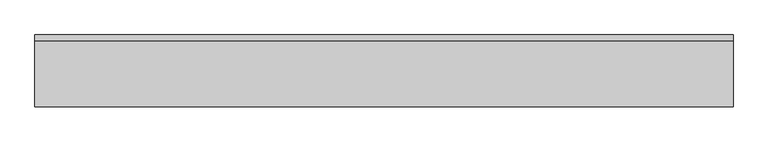
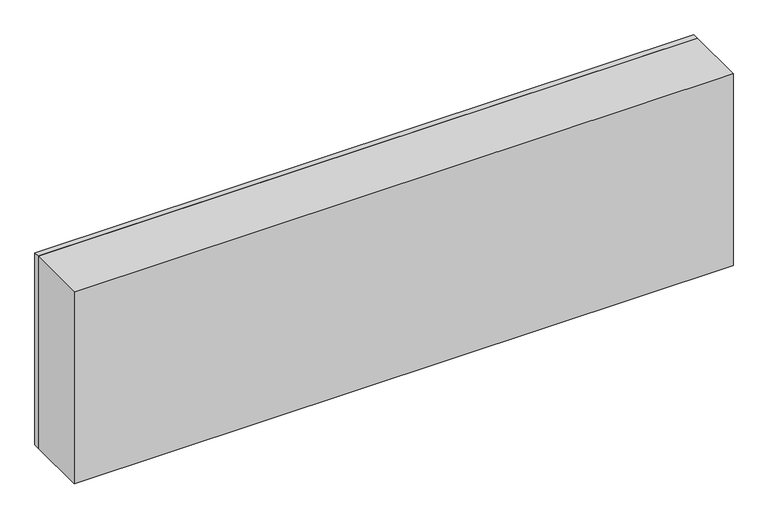
"""IFC4 building model written with IfcOpenShell, lengths in millimetres: furniture geometry, OD_CW_Upper Cabinet : OD_CW_Upper Cabinet."""

from ifc_helpers import new_model, si_unit, frame, origin, place, context, project, spatial, polyline, outline, extrude, source, transform, mapped, element, save


def furniture_bf0ea48e(model_context):
    return source(origin(), model_context, "Body", "SweptSolid", [
        extrude(outline(polyline([(18.7377049, -330.2), (18.7377049, -304.8), (2984.1877049, -304.8), (2984.1877049, -330.2), (18.7377049, -330.2)])), frame((0.0, 0.0, 965.2), z_axis=(0.0, 0.0, 1.0), x_axis=(1.0, 0.0, 0.0)), (0.0, 0.0, 1.0), 914.4),
        extrude(outline(polyline([(18.7377049, -609.6), (18.7377049, -330.2), (2984.1877049, -330.2), (2984.1877049, -609.6), (18.7377049, -609.6)])), frame((0.0, 0.0, 965.2), z_axis=(0.0, 0.0, 1.0), x_axis=(1.0, 0.0, 0.0)), (0.0, 0.0, 1.0), 914.4),
    ])


if __name__ == "__main__":
    model = new_model("IFC4")
    model_context = context("Model", 3, world=origin())
    ifc_project = project(units=[si_unit("LENGTHUNIT", "METRE", prefix="MILLI")], contexts=[model_context])
    site = spatial("IfcSite", under=ifc_project)
    building = spatial("IfcBuilding", under=site)
    placement = place(None, origin())
    furniture_shape = furniture_bf0ea48e(model_context)
    element("IfcFurniture", 1, ObjectType="OD_CW_Upper Cabinet : OD_CW_Upper Cabinet", at=placement, inside=building, context=model_context, shape_type="MappedRepresentation", body=[
        mapped(furniture_shape, transform((0.0, 0.0, 0.0), x_axis=(1.0, 0.0, 0.0), y_axis=(0.0, 1.0, 0.0), z_axis=(0.0, 0.0, 1.0))),
    ])
    save(model, "model.ifc")

# Revit data of these elements
# Type "OD_CW_Upper Cabinet : OD_CW_Upper Cabinet"
#   OD_CW_Width [instance default] = 2' - 2"
#   OD_CW_Off Floor [instance default] = 3' - 2"
#   OD_CW_Length [instance default] = 8' - 0"
#   OD_CW_Height [instance default] = 7' - 0"
#   Depth = 2' - 0"
#   Height = 3' - 0"
#   Width = 4' - 0"
#   OD_CW_Material_Front Panel [instance default] = none
# Element 1 (IfcFurniture, "OD_CW_Upper Cabinet : OD_CW_Upper Cabinet")
#   OD_CW_Width = 1' - 0"
#   OD_CW_Length = 9' - 8 3/4"
#   OD_CW_Height = 3' - 0"
#   Materials on its faces: "casework"
# Materials
#   "casework": class "Generic", colour RGB 229 229 229, transparency 0, Cost = 0
